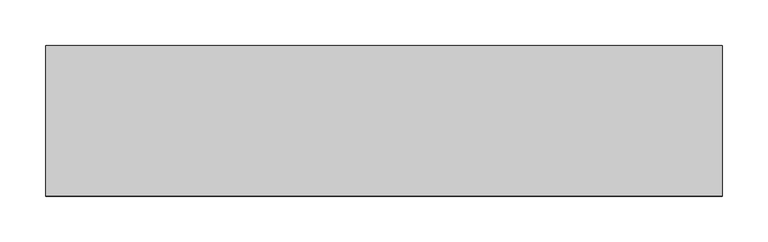
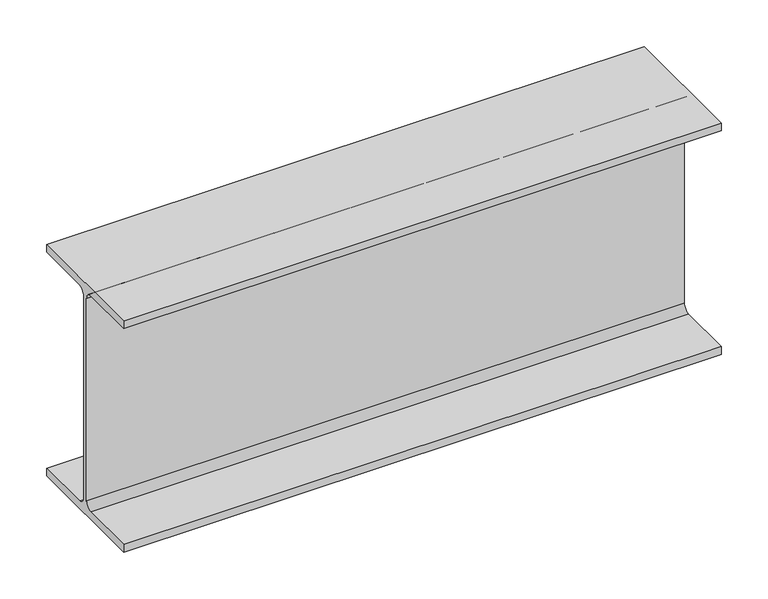
"""IFC4 building model written with IfcOpenShell, lengths in millimetres: beam geometry, Old_Steel Beam_H-KSD3502 : H_SB_ASB_H-300×300x10x15."""

from ifc_helpers import new_model, si_unit, point, frame, frame_2d, origin, place, context, project, spatial, polyline, circle_curve, trimmed, segment, composite_curve, outline, extrude, source, transform, mapped, element, save


def beam_b90b2246(model_context):
    return source(origin(), model_context, "Body", "SweptSolid", [
        extrude(outline(composite_curve([segment(polyline([(82.5, -141.5), (82.5, -151.7), (-82.5, -151.7), (-82.5, -141.5), (-11.9, -141.5)]), True, "CONTINUOUS"), segment(trimmed(circle_curve(frame_2d((-11.9, -132.6)), 8.9), [point((-11.9, -141.5))], [point((-3.0, -132.6))], True, "CARTESIAN"), True, "CONTINUOUS"), segment(polyline([(-3.0, -132.6), (-3.0, 132.6)]), True, "CONTINUOUS"), segment(trimmed(circle_curve(frame_2d((-11.9, 132.6)), 8.9), [point((-3.0, 132.6))], [point((-11.9, 141.5))], True, "CARTESIAN"), True, "CONTINUOUS"), segment(polyline([(-11.9, 141.5), (-82.5, 141.5), (-82.5, 151.7), (82.5, 151.7), (82.5, 141.5), (11.9, 141.5)]), True, "CONTINUOUS"), segment(trimmed(circle_curve(frame_2d((11.9, 132.6)), 8.9), [point((11.9, 141.5))], [point((3.0, 132.6))], True, "CARTESIAN"), True, "CONTINUOUS"), segment(polyline([(3.0, 132.6), (3.0, -132.6)]), True, "CONTINUOUS"), segment(trimmed(circle_curve(frame_2d((11.9, -132.6)), 8.9), [point((3.0, -132.6))], [point((11.9, -141.5))], True, "CARTESIAN"), True, "CONTINUOUS"), segment(polyline([(11.9, -141.5), (82.5, -141.5)]), True, "CONTINUOUS")], self_intersect=False)), frame((-502.4937811, 0.0, 0.0), z_axis=(1.0, 0.0, 0.0), x_axis=(0.0, 1.0, 0.0)), (0.0, 0.0, 1.0), 740.4687108),
    ])


if __name__ == "__main__":
    model = new_model("IFC4")
    model_context = context("Model", 3, world=origin())
    ifc_project = project(units=[si_unit("LENGTHUNIT", "METRE", prefix="MILLI")], contexts=[model_context])
    site = spatial("IfcSite", under=ifc_project)
    building = spatial("IfcBuilding", under=site)
    placement = place(None, origin())
    beam_shape = beam_b90b2246(model_context)
    element("IfcBeam", 1, ObjectType="Old_Steel Beam_H-KSD3502 : H_SB_ASB_H-300×300x10x15", at=placement, inside=building, context=model_context, shape_type="MappedRepresentation", body=[
        mapped(beam_shape, transform((0.0, 0.0, 0.0), x_axis=(1.0, 0.0, 0.0), y_axis=(0.0, 1.0, 0.0), z_axis=(0.0, 0.0, 1.0))),
    ])
    save(model, "model.ifc")

# Revit data of these elements
# Type "Old_Steel Beam_H-KSD3502 : H_SB_ASB_H-300×300x10x15"
#   Width = 30.0 cm
#   Web Thickness = 1.0 cm
#   Web Fillet = 1.8 cm
#   Warping Constant = 1370670.0 cm⁶
#   Torsional Moment of Inertia = 77.00 cm⁴
#   Torsional Modulus = 1.0 cm³
#   Section Area = 119.8 cm²
#   Plastic Modulus weak axis = 684.0 cm³
#   Plastic Modulus strong axis = 1500.0 cm³
#   Perimeter = 1.75 m²/m
#   Nominal Weight = 94.00 kgf/m
#   Moment of Inertia weak axis = 6750.00 cm⁴
#   Moment of Inertia strong axis = 20400.00 cm⁴
#   Height = 30.0 cm
#   Flange Thickness = 1.5 cm
#   Elastic Modulus weak axis = 450.0 cm³
#   Elastic Modulus strong axis = 1360.0 cm³
#   Centroid Vertical = 15.0 cm
#   Centroid Horizontal = 15.0 cm
#   Length [instance default] = 1.5240 m
#   Structural Material [instance default] = Steel, 45-345
#   Assembly Code = ""
# Element 1 (IfcBeam, "Old_Steel Beam_H-KSD3502 : H_SB_ASB_H-300×300x10x15")
#   Structural Material = none
# Materials
#   "Steel, 45-345": class "Metal", colour RGB 189 187 185, transparency 0, Description = "Steel 345 MPa", Cost = 0
